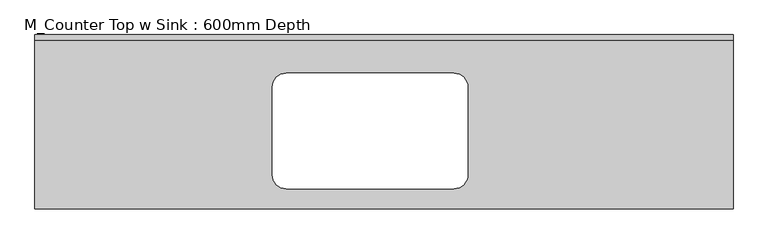
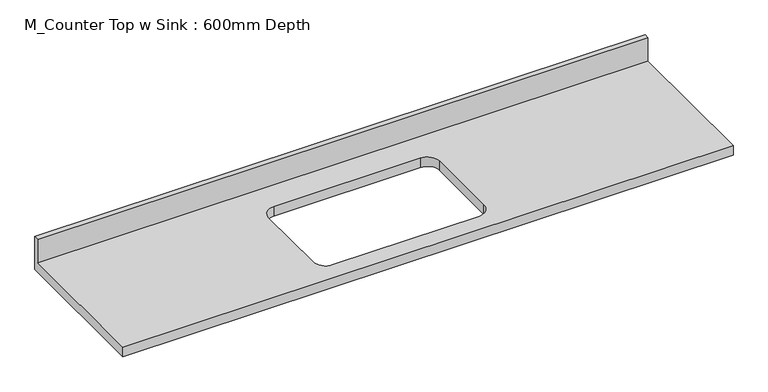
"""IFC4 building model written with IfcOpenShell, lengths in millimetres: furniture geometry, M_Counter Top w Sink : 600mm Depth."""

from ifc_helpers import new_model, si_unit, frame, origin, place, context, project, spatial, polyline, circle_curve, source, transform, mapped, element, save
from ifc_brep_helpers import plane_surface, revolved_surface, advanced_brep


def m_counter_top_w_sink_600mm_depth_b15aa752(model_context):
    return source(origin(), model_context, "Body", "AdvancedBrep", [
        advanced_brep(
        [(-1200.4622951, -625.0, 900.0), (1299.5377049, -625.0, 900.0), (1299.5377049, -19.05, 900.0), (-1200.4622951, -19.05, 900.0), (-299.8622951, -137.3, 900.0), (298.9377049, -137.3, 900.0), (349.7377049, -188.1, 900.0), (349.7377049, -501.9, 900.0), (298.9377049, -552.7, 900.0), (-299.8622951, -552.7, 900.0), (-350.6622951, -501.9, 900.0), (-350.6622951, -188.1, 900.0), (1299.5377049, 0.0, 860.0), (1299.5377049, -625.0, 860.0), (-1200.4622951, -625.0, 860.0), (-1200.4622951, 0.0, 860.0), (298.9377049, -137.3, 860.0), (-299.8622951, -137.3, 860.0), (-350.6622951, -188.1, 860.0), (-350.6622951, -501.9, 860.0), (-299.8622951, -552.7, 860.0), (298.9377049, -552.7, 860.0), (349.7377049, -501.9, 860.0), (349.7377049, -188.1, 860.0), (-1200.4622951, 0.0, 1001.6), (1299.5377049, 0.0, 1001.6), (-1200.4622951, -19.05, 1001.6), (1299.5377049, -19.05, 1001.6)],
        [
            (0, 1),
            (1, 2),
            (2, 3),
            (3, 0),
            (4, 5),
            (5, 6, circle_curve(frame((298.9377049, -188.1, 900.0), z_axis=(0.0, 0.0, -1.0), x_axis=(1.0, 0.0, 0.0)), 50.8)),
            (6, 7),
            (7, 8, circle_curve(frame((298.9377049, -501.9, 900.0), z_axis=(0.0, 0.0, -1.0), x_axis=(1.0, 0.0, 0.0)), 50.8)),
            (8, 9),
            (9, 10, circle_curve(frame((-299.8622951, -501.9, 900.0), z_axis=(0.0, 0.0, -1.0), x_axis=(1.0, 0.0, 0.0)), 50.8)),
            (10, 11),
            (11, 4, circle_curve(frame((-299.8622951, -188.1, 900.0), z_axis=(0.0, 0.0, -1.0), x_axis=(1.0, 0.0, 0.0)), 50.8)),
            (12, 13),
            (13, 14),
            (14, 15),
            (15, 12),
            (16, 17),
            (17, 18, circle_curve(frame((-299.8622951, -188.1, 860.0), z_axis=(0.0, 0.0, 1.0), x_axis=(1.0, 0.0, 0.0)), 50.8)),
            (18, 19),
            (19, 20, circle_curve(frame((-299.8622951, -501.9, 860.0), z_axis=(0.0, 0.0, 1.0), x_axis=(1.0, 0.0, 0.0)), 50.8)),
            (20, 21),
            (21, 22, circle_curve(frame((298.9377049, -501.9, 860.0), z_axis=(0.0, 0.0, 1.0), x_axis=(1.0, 0.0, 0.0)), 50.8)),
            (22, 23),
            (23, 16, circle_curve(frame((298.9377049, -188.1, 860.0), z_axis=(0.0, 0.0, 1.0), x_axis=(1.0, 0.0, 0.0)), 50.8)),
            (15, 24),
            (24, 25),
            (25, 12),
            (14, 0),
            (3, 26),
            (26, 24),
            (13, 1),
            (25, 27),
            (27, 2),
            (26, 27),
            (4, 17),
            (16, 5),
            (11, 18),
            (10, 19),
            (9, 20),
            (8, 21),
            (7, 22),
            (6, 23),
        ],
        [
            plane_surface(frame((-1200.4622951, 0.0, 900.0), z_axis=(0.0, 0.0, 1.0), x_axis=(-1.0, 0.0, 0.0))),
            plane_surface(frame((-1200.4622951, 0.0, 860.0), z_axis=(0.0, 0.0, -1.0), x_axis=(1.0, 0.0, 0.0))),
            plane_surface(frame((1299.5377049, 0.0, 900.0), z_axis=(0.0, 1.0, 0.0), x_axis=(0.0, 0.0, -1.0))),
            plane_surface(frame((-1200.4622951, 0.0, 900.0), z_axis=(-1.0, 0.0, 0.0), x_axis=(0.0, 0.0, -1.0))),
            plane_surface(frame((-1200.4622951, -625.0, 900.0), z_axis=(0.0, -1.0, 0.0), x_axis=(0.0, 0.0, -1.0))),
            plane_surface(frame((1299.5377049, -625.0, 900.0), z_axis=(1.0, 0.0, 0.0), x_axis=(0.0, 0.0, -1.0))),
            plane_surface(frame((-1200.4622951, 0.0, 1001.6), z_axis=(0.0, 0.0, 1.0), x_axis=(0.0, -1.0, 0.0))),
            plane_surface(frame((-1200.4622951, -19.05, 1001.6), z_axis=(0.0, -1.0, 0.0), x_axis=(0.0, 0.0, -1.0))),
            plane_surface(frame((298.9377049, -137.3, 900.0), z_axis=(0.0, -1.0, 0.0), x_axis=(0.0, 0.0, -1.0))),
            revolved_surface(polyline([(-249.06229509999997, -188.1, 900.0), (-249.06229509999997, -188.1, 860.0)]), (-299.8622951, -188.1, 860.0), (0.0, 0.0, 1.0)),
            plane_surface(frame((-350.6622951, -188.1, 900.0), z_axis=(1.0, 0.0, 0.0), x_axis=(0.0, 0.0, -1.0))),
            revolved_surface(polyline([(-249.06229509999997, -501.9, 900.0), (-249.06229509999997, -501.9, 860.0)]), (-299.8622951, -501.9, 860.0), (0.0, 0.0, 1.0)),
            plane_surface(frame((-299.8622951, -552.7, 900.0), z_axis=(0.0, 1.0, 0.0), x_axis=(0.0, 0.0, -1.0))),
            revolved_surface(polyline([(349.73770490000004, -501.9, 900.0), (349.73770490000004, -501.9, 860.0)]), (298.9377049, -501.9, 860.0), (0.0, 0.0, 1.0)),
            plane_surface(frame((349.7377049, -501.9, 900.0), z_axis=(-1.0, 0.0, 0.0), x_axis=(0.0, 0.0, -1.0))),
            revolved_surface(polyline([(349.73770490000004, -188.1, 900.0), (349.73770490000004, -188.1, 860.0)]), (298.9377049, -188.1, 860.0), (0.0, 0.0, 1.0)),
        ],
        [
            (0, [[1, 2, 3, 4], [5, 6, 7, 8, 9, 10, 11, 12]]),
            (1, [[13, 14, 15, 16], [17, 18, 19, 20, 21, 22, 23, 24]]),
            (2, [[-16, 25, 26, 27]]),
            (3, [[-15, 28, -4, 29, 30, -25]]),
            (4, [[-1, -28, -14, 31]]),
            (5, [[-13, -27, 32, 33, -2, -31]]),
            (6, [[-30, 34, -32, -26]]),
            (7, [[-34, -29, -3, -33]]),
            (8, [[35, -17, 36, -5]]),
            (9, [[-35, -12, 37, -18]]),
            (10, [[-37, -11, 38, -19]]),
            (11, [[-38, -10, 39, -20]]),
            (12, [[-39, -9, 40, -21]]),
            (13, [[-40, -8, 41, -22]]),
            (14, [[-41, -7, 42, -23]]),
            (15, [[-36, -24, -42, -6]]),
        ],
    ),
    ])


if __name__ == "__main__":
    model = new_model("IFC4")
    model_context = context("Model", 3, world=origin())
    ifc_project = project(units=[si_unit("LENGTHUNIT", "METRE", prefix="MILLI")], contexts=[model_context])
    site = spatial("IfcSite", under=ifc_project)
    building = spatial("IfcBuilding", under=site)
    placement = place(None, origin())
    m_counter_top_w_sink_600mm_depth_shape = m_counter_top_w_sink_600mm_depth_b15aa752(model_context)
    element("IfcFurniture", 1, ObjectType="M_Counter Top w Sink : 600mm Depth", at=placement, inside=building, context=model_context, shape_type="MappedRepresentation", body=[
        mapped(m_counter_top_w_sink_600mm_depth_shape, transform((0.0, 0.0, 0.0), x_axis=(1.0, 0.0, 0.0), y_axis=(0.0, 1.0, 0.0), z_axis=(0.0, 0.0, 1.0))),
    ])
    save(model, "model.ifc")

# Revit data of these elements
# Type "M_Counter Top w Sink : 600mm Depth"
#   Counter Thickness = 0.04 m
#   Depth = 0.625 m
#   Height = 0.90 m
#   Length [instance default] = 2.50 m
#   Sink Location [instance default] = 1.20 m
#   Sink Location To Wall [instance default] = 0.15 m
#   Sink Opening Depth [instance default] = 0.39 m
#   Sink Opening Width [instance default] = 0.675 m
#   Counter Top Material = none
# Element 1 (IfcFurniture, "M_Counter Top w Sink : 600mm Depth")
#   Materials on its faces: "Counter Top"
# Materials
#   "Counter Top": class "Wood", colour RGB 226 177 128, transparency 0
